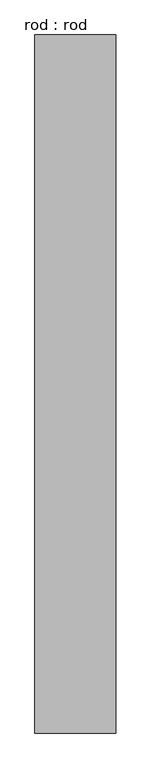
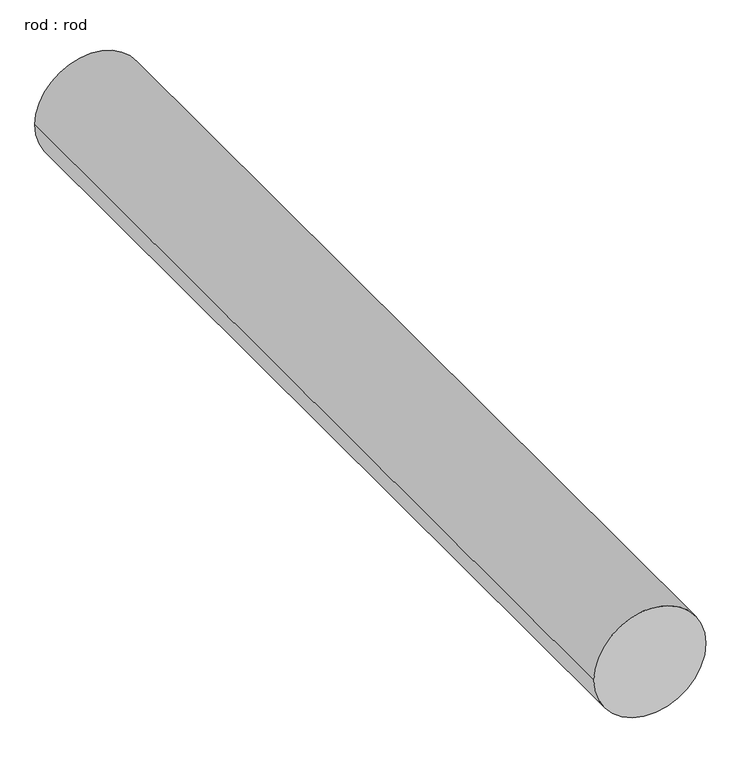
"""IFC4 building model written with IfcOpenShell, lengths in millimetres: proxy geometry, rod : rod."""

from ifc_helpers import new_model, si_unit, point, frame, frame_2d, origin, place, context, project, spatial, circle_curve, trimmed, segment, composite_curve, outline, extrude, source, transform, mapped, element, save


def rod_rod_8a4bef2b(model_context):
    return source(origin(), model_context, "Body", "SweptSolid", [
        extrude(outline(composite_curve([segment(trimmed(circle_curve(frame_2d((0.0108462, 0.0)), 200.0), [point((0.0108462, 200.0))], [point((0.0108462, -200.0))], False, "CARTESIAN"), True, "CONTINUOUS"), segment(trimmed(circle_curve(frame_2d((0.0108462, 0.0)), 200.0), [point((0.0108462, -200.0))], [point((0.0108462, 200.0))], False, "CARTESIAN"), True, "CONTINUOUS")], self_intersect=False)), frame((0.0, 2362.7286153, 0.0), z_axis=(0.0, 1.0, 0.0), x_axis=(0.0, 0.0, 1.0)), (0.0, 0.0, 1.0), 3460.0),
    ])


if __name__ == "__main__":
    model = new_model("IFC4")
    model_context = context("Model", 3, world=origin())
    ifc_project = project(units=[si_unit("LENGTHUNIT", "METRE", prefix="MILLI")], contexts=[model_context])
    site = spatial("IfcSite", under=ifc_project)
    building = spatial("IfcBuilding", under=site)
    placement = place(None, origin())
    rod_rod_shape = rod_rod_8a4bef2b(model_context)
    element("IfcBuildingElementProxy", 1, Name="rod : rod", ObjectType="rod : rod", at=placement, inside=building, context=model_context, shape_type="MappedRepresentation", body=[
        mapped(rod_rod_shape, transform((0.0, 0.0, 0.0), x_axis=(1.0, 0.0, 0.0), y_axis=(0.0, 1.0, 0.0), z_axis=(0.0, 0.0, 1.0))),
    ])
    save(model, "model.ifc")

# Revit data of these elements
# Type "rod : rod"
#   Default Elevation = 0
